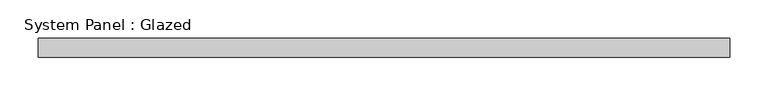
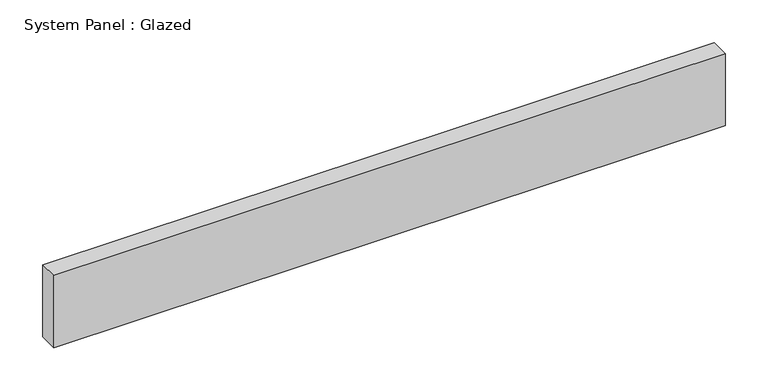
"""IFC4 building model written with IfcOpenShell, lengths in millimetres: plate geometry, System Panel : Glazed."""

from ifc_helpers import new_model, si_unit, origin, origin_with_axes, place, context, project, spatial, polyline, outline, extrude, source, transform, mapped, element, save


def system_panel_glazed_7330a8e7(model_context):
    return source(origin(), model_context, "Body", "SweptSolid", [
        extrude(outline(polyline([(451.2500002, 24.5), (-451.2500002, 24.5), (-451.2500002, 49.5), (451.2500002, 49.5), (451.2500002, 24.5)])), origin_with_axes(), (0.0, 0.0, 1.0), 102.5),
    ])


if __name__ == "__main__":
    model = new_model("IFC4")
    model_context = context("Model", 3, world=origin())
    ifc_project = project(units=[si_unit("LENGTHUNIT", "METRE", prefix="MILLI")], contexts=[model_context])
    site = spatial("IfcSite", under=ifc_project)
    building = spatial("IfcBuilding", under=site)
    placement = place(None, origin())
    system_panel_glazed_shape = system_panel_glazed_7330a8e7(model_context)
    element("IfcPlate", 1, ObjectType="System Panel : Glazed", at=placement, inside=building, context=model_context, shape_type="MappedRepresentation", body=[
        mapped(system_panel_glazed_shape, transform((0.0, 0.0, 0.0), x_axis=(1.0, 0.0, 0.0), y_axis=(0.0, 1.0, 0.0), z_axis=(0.0, 0.0, 1.0))),
    ])
    save(model, "model.ifc")

# Revit data of these elements
# Type "System Panel : Glazed"
#   Construction Type Id = "GSP4R"
#   Analytic Construction = "1/8 in Pilkington single glazing"
#   Visual Light Transmittance = 0.9
#   Solar Heat Gain Coefficient = 0.86
#   Heat Transfer Coefficient (U) = 6.7069 W/(m²·K)
#   Define Thermal Properties by = 1
# Element 1 (IfcPlate, "System Panel : Glazed")
#   Materials on its faces: "Glass"
# Materials
#   "Glass": class "Glass", colour RGB 245 245 243, transparency 1, Description = "Soda Lime Glass", Cost = 0
